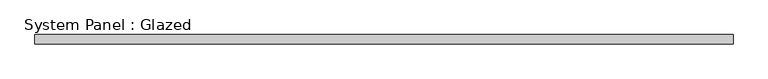
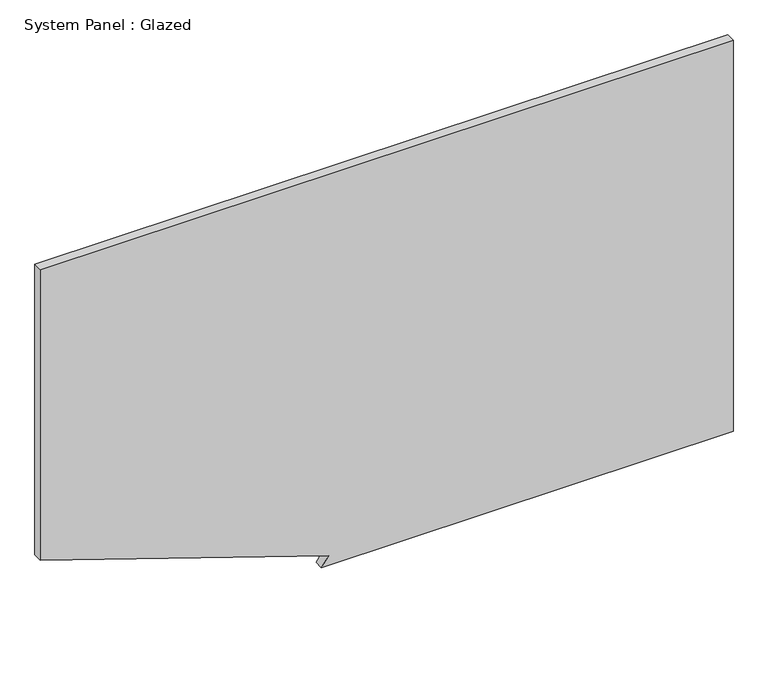
"""IFC4 building model written with IfcOpenShell, lengths in millimetres: plate geometry, System Panel : Glazed."""

from ifc_helpers import new_model, si_unit, frame, origin, place, context, project, spatial, polyline, outline, extrude, source, transform, mapped, element, save


def system_panel_glazed_a1864e1b(model_context):
    return source(origin(), model_context, "Body", "SweptSolid", [
        extrude(outline(polyline([(0.0, -182.3127692), (0.0, 968.375), (1155.7, 968.375), (1155.7, -968.375), (297.2056207, -968.375), (28.4913894, -162.232306), (0.0, -182.3127692)])), frame((0.0, -44.45, 0.0), z_axis=(0.0, 1.0, 0.0), x_axis=(0.0, 0.0, 1.0)), (0.0, 0.0, 1.0), 25.4),
    ])


if __name__ == "__main__":
    model = new_model("IFC4")
    model_context = context("Model", 3, world=origin())
    ifc_project = project(units=[si_unit("LENGTHUNIT", "METRE", prefix="MILLI")], contexts=[model_context])
    site = spatial("IfcSite", under=ifc_project)
    building = spatial("IfcBuilding", under=site)
    placement = place(None, origin())
    system_panel_glazed_shape = system_panel_glazed_a1864e1b(model_context)
    element("IfcPlate", 1, ObjectType="System Panel : Glazed", at=placement, inside=building, context=model_context, shape_type="MappedRepresentation", body=[
        mapped(system_panel_glazed_shape, transform((0.0, 0.0, 0.0), x_axis=(1.0, 0.0, 0.0), y_axis=(0.0, 1.0, 0.0), z_axis=(0.0, 0.0, 1.0))),
    ])
    save(model, "model.ifc")

# Revit data of these elements
# Element 1 (IfcPlate, "System Panel : Glazed")
#   Materials on its faces: "Glass"
# Materials
#   "Glass": class "Glass", colour RGB 0 128 192, transparency 0.75
